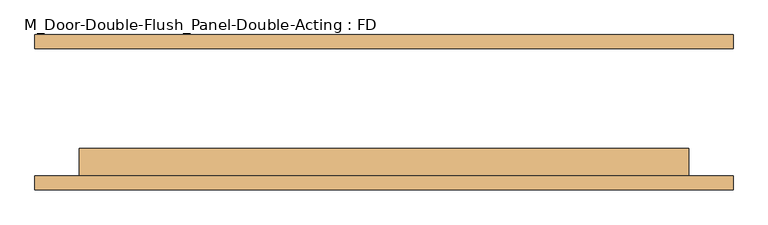
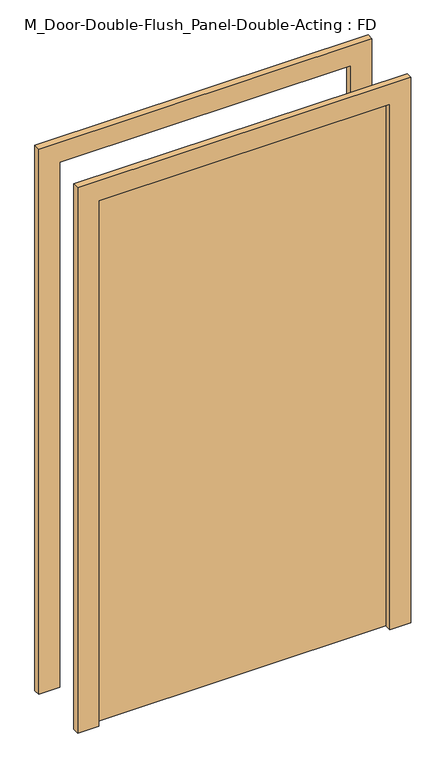
"""IFC4 building model written with IfcOpenShell, lengths in millimetres: door geometry, M_Door-Double-Flush_Panel-Double-Acting : FD."""

from ifc_helpers import new_model, si_unit, frame, origin, origin_with_axes, place, context, project, spatial, polyline, outline, extrude, source, transform, mapped, element, save


def m_door_double_flush_panel_double_acting_fd_77c7f73a(model_context):
    return source(origin(), model_context, "Body", "SweptSolid", [
        extrude(outline(polyline([(2180.0, -630.0), (0.0, -630.0), (0.0, -550.0), (2100.0, -550.0), (2100.0, 550.0), (0.0, 550.0), (0.0, 630.0), (2180.0, 630.0), (2180.0, -630.0)])), frame((0.0, -140.0, 0.0), z_axis=(0.0, 1.0, 0.0), x_axis=(0.0, 0.0, 1.0)), (0.0, 0.0, 1.0), 25.0),
        extrude(outline(polyline([(2100.0, -550.0), (2100.0, 550.0), (0.0, 550.0), (0.0, 630.0), (2180.0, 630.0), (2180.0, -630.0), (0.0, -630.0), (0.0, -550.0), (2100.0, -550.0)])), frame((0.0, 115.0, 0.0), z_axis=(0.0, 1.0, 0.0), x_axis=(0.0, 0.0, 1.0)), (0.0, 0.0, 1.0), 25.0),
        extrude(outline(polyline([(-550.0, -115.0), (-550.0, -65.0), (550.0, -65.0), (550.0, -115.0), (-550.0, -115.0)])), origin_with_axes(), (0.0, 0.0, 1.0), 2100.0),
    ])


if __name__ == "__main__":
    model = new_model("IFC4")
    model_context = context("Model", 3, world=origin())
    ifc_project = project(units=[si_unit("LENGTHUNIT", "METRE", prefix="MILLI")], contexts=[model_context])
    site = spatial("IfcSite", under=ifc_project)
    building = spatial("IfcBuilding", under=site)
    placement = place(None, origin())
    m_door_double_flush_panel_double_acting_fd_shape = m_door_double_flush_panel_double_acting_fd_77c7f73a(model_context)
    element("IfcDoor", 1, ObjectType="M_Door-Double-Flush_Panel-Double-Acting : FD", at=placement, inside=building, context=model_context, shape_type="MappedRepresentation", body=[
        mapped(m_door_double_flush_panel_double_acting_fd_shape, transform((0.0, 0.0, 0.0), x_axis=(1.0, 0.0, 0.0), y_axis=(0.0, 1.0, 0.0), z_axis=(0.0, 0.0, 1.0))),
    ])
    save(model, "model.ifc")

# Revit data of these elements
# Type "M_Door-Double-Flush_Panel-Double-Acting : FD"
#   Type Mark = "55"
#   Construction Type Id = "DOOR"
#   Assembly Code = "C1020"
#   Analytic Construction = "Wooden"
#   W = 55 cm
#   Thickness = 5 cm
#   Thermal Resistance (R) = 0.455703 (m²·K)/W
#   Swing Angle [instance default] = 90.00°
#   Heat Transfer Coefficient (U) = 2.19465 W/(m²·K)
#   Height = 210 cm
#   Trim Projection Ext. = 2.5 cm
#   Trim Projection Int. = 2.5 cm
#   Trim Width Ext. = 8 cm
#   Trim Width Int. = 8 cm
#   Width = 110 cm
#   Panel Material = Wood - Birch - Solid Stained Light Low Gloss
#   Trim Material = Paint - Sienna
#   Visual Light Transmittance = 0
#   Solar Heat Gain Coefficient = 0
#   Function = (empty or 0)
#   Wall Closure = (empty or 0)
# Element 1 (IfcDoor, "M_Door-Double-Flush_Panel-Double-Acting : FD")
#   Materials on its faces: "Paint - Sienna", "Wood - Birch - Solid Stained Light Low Gloss"
# Materials
#   "Wood - Birch - Solid Stained Light Low Gloss": class "Wood", colour RGB 210 159 95, transparency 0, Cost = 0
#   "Paint - Sienna": class "Miscellaneous", colour RGB 118 70 51, transparency 0, Cost = 0
